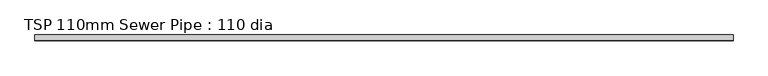
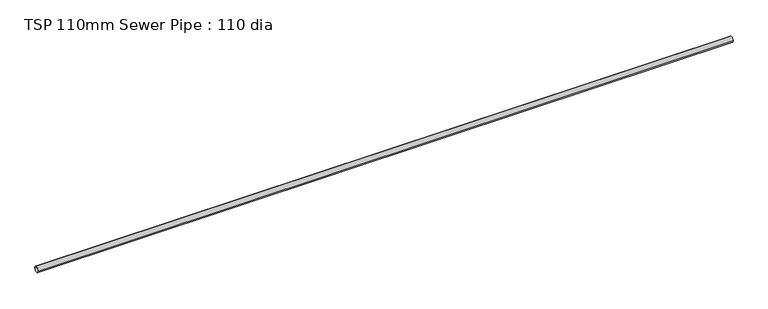
"""IFC4 building model written with IfcOpenShell, lengths in millimetres: flow terminal geometry, TSP 110mm Sewer Pipe : 110 dia."""

import ifcopenshell
import ifcopenshell.guid

model = None  # the IFC model being written
_history = None  # IfcOwnerHistory: only IFC2X3 demands one
_inside = {}  # id of a spatial element -> (the spatial element, [elements in it])
_under = {}  # id of a project, library or spatial element -> (it, [spatial elements below it])
_declared = {}  # id of a project -> (the project, [libraries it declares])
_typed = {}  # id of a type object -> (the type object, [elements of that type])
_made_of = {}  # id of a material, layer set ... -> (it, [elements and type objects made of it])


def new_model(schema):
    """Start an empty IFC model of exactly this schema.

    Asked for "IFC4X3", IfcOpenShell would pick the latest addendum, in which some entities
    have other attributes; the version numbers below select the first issue.
    IFC2X3 requires an IfcOwnerHistory on every rooted entity: one is made here for all.
    """
    global model, _history
    if schema == "IFC4X3":
        model = ifcopenshell.file(schema_version=(4, 3, 0, 0))
    else:
        model = ifcopenshell.file(schema=schema)
    _inside.clear()
    _under.clear()
    _declared.clear()
    _typed.clear()
    _made_of.clear()
    _history = None
    if model.schema == "IFC2X3":
        org = make("IfcOrganization", Name="unknown")
        user = make(
            "IfcPersonAndOrganization",
            ThePerson=make("IfcPerson", FamilyName="unknown"),
            TheOrganization=org,
        )
        app = make(
            "IfcApplication",
            ApplicationDeveloper=org,
            Version="unknown",
            ApplicationFullName="unknown",
            ApplicationIdentifier="unknown",
        )
        _history = make(
            "IfcOwnerHistory",
            OwningUser=user,
            OwningApplication=app,
            ChangeAction="ADDED",
            CreationDate=0,
        )
    return model


def make(cls, **values):
    """One entity of the class cls with the attributes given. An attribute that is None is left unset."""
    return model.create_entity(
        cls, **{name: value for name, value in values.items() if value is not None}
    )


def rooted(cls, **values):
    """An entity with a GlobalId (a new one), such as an element, a storey or a relation."""
    return make(cls, GlobalId=ifcopenshell.guid.new(), OwnerHistory=_history, **values)


def si_unit(unit_type, name, prefix=None):
    """IfcSIUnit, for example si_unit("LENGTHUNIT", "METRE", prefix="MILLI")."""
    return make("IfcSIUnit", UnitType=unit_type, Prefix=prefix, Name=name)


def assignment(units):
    """IfcUnitAssignment: the units of a project."""
    return None if units is None else make("IfcUnitAssignment", Units=units)


def point(xyz):
    """IfcCartesianPoint."""
    return None if xyz is None else make("IfcCartesianPoint", Coordinates=xyz)


def direction(xyz):
    """IfcDirection."""
    return None if xyz is None else make("IfcDirection", DirectionRatios=xyz)


def frame(location, z_axis=None, x_axis=None):
    """IfcAxis2Placement3D, a coordinate frame: its origin and axes. An axis left out is left unset."""
    return make(
        "IfcAxis2Placement3D",
        Location=point(location),
        Axis=direction(z_axis),
        RefDirection=direction(x_axis),
    )


def frame_2d(location, x_axis=None):
    """IfcAxis2Placement2D, a coordinate frame in the plane: its origin and x axis."""
    return make(
        "IfcAxis2Placement2D", Location=point(location), RefDirection=direction(x_axis)
    )


def origin():
    """The frame at (0, 0, 0) with its axes left unset."""
    return frame((0.0, 0.0, 0.0))


def origin_2d():
    """The frame at (0, 0) in the plane with its x axis left unset."""
    return frame_2d((0.0, 0.0))


def place(relative_to, where):
    """IfcLocalPlacement: puts the frame where relative to a parent placement (None: the world)."""
    return make(
        "IfcLocalPlacement", PlacementRelTo=relative_to, RelativePlacement=where
    )


def context(
    kind, dimensions, precision=None, world=None, true_north=None, identifier=None
):
    """IfcGeometricRepresentationContext, for example the 3D "Model" context."""
    return make(
        "IfcGeometricRepresentationContext",
        ContextIdentifier=identifier,
        ContextType=kind,
        CoordinateSpaceDimension=dimensions,
        Precision=precision,
        WorldCoordinateSystem=world,
        TrueNorth=true_north,
    )


def project(units=None, contexts=None):
    """IfcProject with its units and contexts."""
    return rooted(
        "IfcProject",
        Name="project",
        RepresentationContexts=contexts,
        UnitsInContext=assignment(units),
    )


def spatial(cls, under=None, at=None, **own):
    """A site, building, storey or space (cls), placed at a placement, below another one or the project."""
    s = rooted(cls, ObjectPlacement=at, **own)
    if under is not None:
        _under.setdefault(under.id(), (under, []))[1].append(s)
    return s


def circle_curve(where, radius):
    """IfcCircle in the frame where."""
    return make("IfcCircle", Position=where, Radius=radius)


def trimmed(basis, trim1, trim2, sense, master):
    """IfcTrimmedCurve: the piece of a basis curve between two trims."""
    return make(
        "IfcTrimmedCurve",
        BasisCurve=basis,
        Trim1=trim1,
        Trim2=trim2,
        SenseAgreement=sense,
        MasterRepresentation=master,
    )


def segment(curve, same_sense, transition):
    """IfcCompositeCurveSegment."""
    return make(
        "IfcCompositeCurveSegment",
        Transition=transition,
        SameSense=same_sense,
        ParentCurve=curve,
    )


def composite_curve(segments, self_intersect=None):
    """IfcCompositeCurve: segments joined end to end."""
    return make("IfcCompositeCurve", Segments=segments, SelfIntersect=self_intersect)


def outline(outer, holes=None, kind="AREA"):
    """IfcArbitraryClosedProfileDef: a profile drawn as a closed curve; with holes, ...WithVoids."""
    if holes is None:
        return make("IfcArbitraryClosedProfileDef", ProfileType=kind, OuterCurve=outer)
    return make(
        "IfcArbitraryProfileDefWithVoids",
        ProfileType=kind,
        OuterCurve=outer,
        InnerCurves=holes,
    )


def extrude(swept, where, along, depth):
    """IfcExtrudedAreaSolid: the profile swept, set in the frame where, extruded along a direction by depth."""
    return make(
        "IfcExtrudedAreaSolid",
        SweptArea=swept,
        Position=where,
        ExtrudedDirection=direction(along),
        Depth=depth,
    )


def shape(context_of_items, identifier, shape_type, items):
    """IfcShapeRepresentation: the items that make up one representation, for example the "Body"."""
    return make(
        "IfcShapeRepresentation",
        ContextOfItems=context_of_items,
        RepresentationIdentifier=identifier,
        RepresentationType=shape_type,
        Items=items,
    )


def source(mapping_origin, context_of_items, identifier, shape_type, items):
    """IfcRepresentationMap: a shape defined once, which mapped items show again and again."""
    return make(
        "IfcRepresentationMap",
        MappingOrigin=mapping_origin,
        MappedRepresentation=shape(context_of_items, identifier, shape_type, items),
    )


def transform(
    local_origin,
    x_axis=None,
    y_axis=None,
    z_axis=None,
    scale=None,
    scale2=None,
    scale3=None,
    uniform=True,
):
    """IfcCartesianTransformationOperator3D, or its non-uniform kind. x_axis, y_axis, z_axis: its Axis1, 2, 3."""
    if uniform:
        return make(
            "IfcCartesianTransformationOperator3D",
            Axis1=direction(x_axis),
            Axis2=direction(y_axis),
            LocalOrigin=point(local_origin),
            Scale=scale,
            Axis3=direction(z_axis),
        )
    return make(
        "IfcCartesianTransformationOperator3DnonUniform",
        Axis1=direction(x_axis),
        Axis2=direction(y_axis),
        LocalOrigin=point(local_origin),
        Scale=scale,
        Axis3=direction(z_axis),
        Scale2=scale2,
        Scale3=scale3,
    )


def mapped(mapping_source, mapping_target):
    """IfcMappedItem: shows the shape of a source again, moved by a transform."""
    return make(
        "IfcMappedItem", MappingSource=mapping_source, MappingTarget=mapping_target
    )


def made_of(thing, what):
    """Note that an element or type object is made of a material, layer set ...; save() writes the relation."""
    if what is not None:
        _made_of.setdefault(what.id(), (what, []))[1].append(thing)
    return thing


def element(
    cls,
    number,
    at=None,
    inside=None,
    cuts=None,
    type_object=None,
    material=None,
    context=None,
    identifier="Body",
    shape_type=None,
    held_by="IfcProductDefinitionShape",
    body=None,
    shapes=None,
    **own,
):
    """One element of the class cls, such as IfcWall. Its Tag is "e" and its number.

    at: its placement. inside: the storey or other place that contains it. cuts: it is an
    opening in that element (IfcRelVoidsElement). A single representation is given by context,
    identifier, shape_type and body (its items); several are given by shapes. held_by: the class
    of the entity that holds the representations. save() writes the other relations.
    """
    e = rooted(cls, Tag="e%d" % number, ObjectPlacement=at, **own)
    if body is not None:
        shapes = [shape(context, identifier, shape_type, body)]
    if shapes is not None:
        e.Representation = make(held_by, Representations=shapes)
    if inside is not None:
        _inside.setdefault(inside.id(), (inside, []))[1].append(e)
    if cuts is not None:
        rooted(
            "IfcRelVoidsElement", RelatingBuildingElement=cuts, RelatedOpeningElement=e
        )
    if type_object is not None:
        _typed.setdefault(type_object.id(), (type_object, []))[1].append(e)
    return made_of(e, material)


def aggregate(whole, parts):
    """IfcRelAggregates: a whole, such as a stair, and the parts it consists of."""
    return rooted("IfcRelAggregates", RelatingObject=whole, RelatedObjects=parts)


def save(model, path):
    """Write the relations noted so far, then the file.

    IfcRelAggregates (storeys below a building ...), IfcRelContainedInSpatialStructure (elements
    in a storey), IfcRelDefinesByType, IfcRelAssociatesMaterial and IfcRelDeclares: one each for
    every whole, place, type object, material and project.
    """
    for whole, parts in _under.values():
        aggregate(whole, parts)
    for where, things in _inside.values():
        rooted(
            "IfcRelContainedInSpatialStructure",
            RelatedElements=things,
            RelatingStructure=where,
        )
    for kind, things in _typed.values():
        rooted("IfcRelDefinesByType", RelatedObjects=things, RelatingType=kind)
    for what, things in _made_of.values():
        rooted("IfcRelAssociatesMaterial", RelatedObjects=things, RelatingMaterial=what)
    for by, libraries in _declared.values():
        rooted("IfcRelDeclares", RelatingContext=by, RelatedDefinitions=libraries)
    model.write(path)


def tsp_110mm_sewer_pipe_110_dia_5c8f30d4(model_context):
    return source(origin(), model_context, "Body", "SweptSolid", [
        extrude(outline(composite_curve([segment(trimmed(circle_curve(origin_2d(), 55.0), [point((-55.0, 0.0))], [point((55.0, 0.0))], False, "CARTESIAN"), True, "CONTINUOUS"), segment(trimmed(circle_curve(origin_2d(), 55.0), [point((55.0, 0.0))], [point((-55.0, 0.0))], False, "CARTESIAN"), True, "CONTINUOUS")], self_intersect=False), holes=[composite_curve([segment(trimmed(circle_curve(origin_2d(), 52.0), [point((-52.0, 0.0))], [point((52.0, 0.0))], True, "CARTESIAN"), True, "CONTINUOUS"), segment(trimmed(circle_curve(origin_2d(), 52.0), [point((52.0, 0.0))], [point((-52.0, 0.0))], True, "CARTESIAN"), True, "CONTINUOUS")], self_intersect=False)]), frame((0.0, 0.0, 0.0), z_axis=(1.0, 0.0, 0.0), x_axis=(0.0, 1.0, 0.0)), (0.0, 0.0, 1.0), 13300.0),
    ])


if __name__ == "__main__":
    model = new_model("IFC4")
    model_context = context("Model", 3, world=origin())
    ifc_project = project(units=[si_unit("LENGTHUNIT", "METRE", prefix="MILLI")], contexts=[model_context])
    site = spatial("IfcSite", under=ifc_project)
    building = spatial("IfcBuilding", under=site)
    placement = place(None, origin())
    tsp_110mm_sewer_pipe_110_dia_shape = tsp_110mm_sewer_pipe_110_dia_5c8f30d4(model_context)
    element("IfcFlowTerminal", 1, ObjectType="TSP 110mm Sewer Pipe : 110 dia", at=placement, inside=building, context=model_context, shape_type="MappedRepresentation", body=[
        mapped(tsp_110mm_sewer_pipe_110_dia_shape, transform((0.0, 0.0, 0.0), x_axis=(1.0, 0.0, 0.0), y_axis=(0.0, 1.0, 0.0), z_axis=(0.0, 0.0, 1.0))),
    ])
    save(model, "model.ifc")

# Revit data of these elements
# Type "TSP 110mm Sewer Pipe : 110 dia"
#   Model = "TSP_110SWB"
#   Model = "TSP_110SWB"
#   Pipe length [instance default] = 1200 mm
#   Pipe dia = 110 mm
#   built-in parameter 1001306 [instance default] = 3.93701 (stored number, unit not read)
#   Default Elevation = 0
# Element 1 (IfcFlowTerminal, "TSP 110mm Sewer Pipe : 110 dia")
#   Pipe length = 13300 mm
#   built-in parameter 1001306 = 43.6352 (stored number, unit not read)
#   Materials on its faces: "Laminate, Brown, Matte"
# Materials
#   "Laminate, Brown, Matte": class "Plastic", colour RGB 128 64 0, transparency 0, Description = "Plastic Laminate - Red, Matte", Cost = 0
